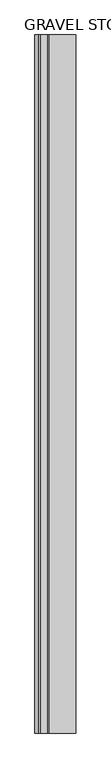
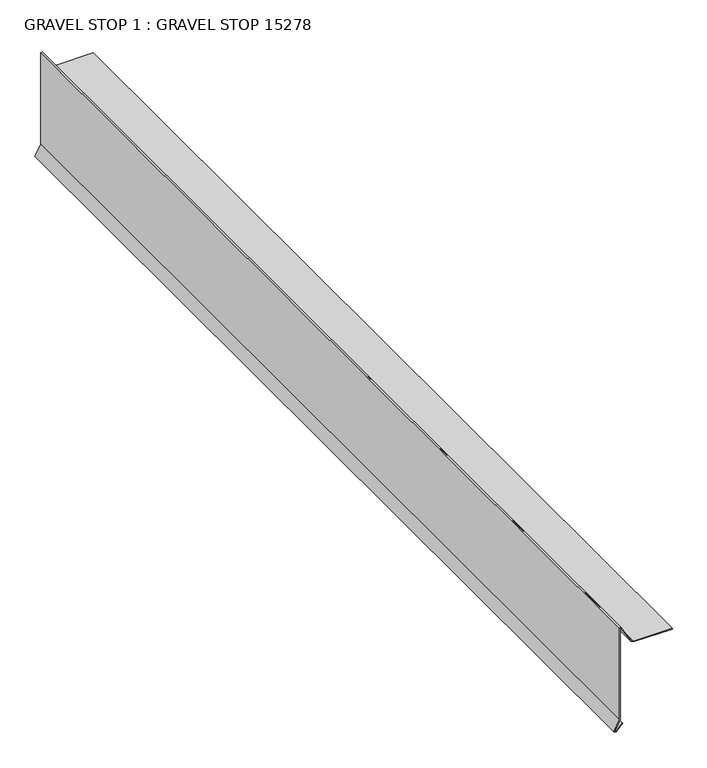
"""IFC4 building model written with IfcOpenShell, lengths in millimetres: proxy geometry, GRAVEL STOP 1 : GRAVEL STOP 15278."""

import ifcopenshell
import ifcopenshell.guid

model = None  # the IFC model being written
_history = None  # IfcOwnerHistory: only IFC2X3 demands one
_inside = {}  # id of a spatial element -> (the spatial element, [elements in it])
_under = {}  # id of a project, library or spatial element -> (it, [spatial elements below it])
_declared = {}  # id of a project -> (the project, [libraries it declares])
_typed = {}  # id of a type object -> (the type object, [elements of that type])
_made_of = {}  # id of a material, layer set ... -> (it, [elements and type objects made of it])


def new_model(schema):
    """Start an empty IFC model of exactly this schema.

    Asked for "IFC4X3", IfcOpenShell would pick the latest addendum, in which some entities
    have other attributes; the version numbers below select the first issue.
    IFC2X3 requires an IfcOwnerHistory on every rooted entity: one is made here for all.
    """
    global model, _history
    if schema == "IFC4X3":
        model = ifcopenshell.file(schema_version=(4, 3, 0, 0))
    else:
        model = ifcopenshell.file(schema=schema)
    _inside.clear()
    _under.clear()
    _declared.clear()
    _typed.clear()
    _made_of.clear()
    _history = None
    if model.schema == "IFC2X3":
        org = make("IfcOrganization", Name="unknown")
        user = make(
            "IfcPersonAndOrganization",
            ThePerson=make("IfcPerson", FamilyName="unknown"),
            TheOrganization=org,
        )
        app = make(
            "IfcApplication",
            ApplicationDeveloper=org,
            Version="unknown",
            ApplicationFullName="unknown",
            ApplicationIdentifier="unknown",
        )
        _history = make(
            "IfcOwnerHistory",
            OwningUser=user,
            OwningApplication=app,
            ChangeAction="ADDED",
            CreationDate=0,
        )
    return model


def make(cls, **values):
    """One entity of the class cls with the attributes given. An attribute that is None is left unset."""
    return model.create_entity(
        cls, **{name: value for name, value in values.items() if value is not None}
    )


def rooted(cls, **values):
    """An entity with a GlobalId (a new one), such as an element, a storey or a relation."""
    return make(cls, GlobalId=ifcopenshell.guid.new(), OwnerHistory=_history, **values)


def si_unit(unit_type, name, prefix=None):
    """IfcSIUnit, for example si_unit("LENGTHUNIT", "METRE", prefix="MILLI")."""
    return make("IfcSIUnit", UnitType=unit_type, Prefix=prefix, Name=name)


def assignment(units):
    """IfcUnitAssignment: the units of a project."""
    return None if units is None else make("IfcUnitAssignment", Units=units)


def point(xyz):
    """IfcCartesianPoint."""
    return None if xyz is None else make("IfcCartesianPoint", Coordinates=xyz)


def direction(xyz):
    """IfcDirection."""
    return None if xyz is None else make("IfcDirection", DirectionRatios=xyz)


def frame(location, z_axis=None, x_axis=None):
    """IfcAxis2Placement3D, a coordinate frame: its origin and axes. An axis left out is left unset."""
    return make(
        "IfcAxis2Placement3D",
        Location=point(location),
        Axis=direction(z_axis),
        RefDirection=direction(x_axis),
    )


def origin():
    """The frame at (0, 0, 0) with its axes left unset."""
    return frame((0.0, 0.0, 0.0))


def place(relative_to, where):
    """IfcLocalPlacement: puts the frame where relative to a parent placement (None: the world)."""
    return make(
        "IfcLocalPlacement", PlacementRelTo=relative_to, RelativePlacement=where
    )


def context(
    kind, dimensions, precision=None, world=None, true_north=None, identifier=None
):
    """IfcGeometricRepresentationContext, for example the 3D "Model" context."""
    return make(
        "IfcGeometricRepresentationContext",
        ContextIdentifier=identifier,
        ContextType=kind,
        CoordinateSpaceDimension=dimensions,
        Precision=precision,
        WorldCoordinateSystem=world,
        TrueNorth=true_north,
    )


def project(units=None, contexts=None):
    """IfcProject with its units and contexts."""
    return rooted(
        "IfcProject",
        Name="project",
        RepresentationContexts=contexts,
        UnitsInContext=assignment(units),
    )


def spatial(cls, under=None, at=None, **own):
    """A site, building, storey or space (cls), placed at a placement, below another one or the project."""
    s = rooted(cls, ObjectPlacement=at, **own)
    if under is not None:
        _under.setdefault(under.id(), (under, []))[1].append(s)
    return s


def polyline(points):
    """IfcPolyline through the points."""
    return make("IfcPolyline", Points=[point(p) for p in points])


def outline(outer, holes=None, kind="AREA"):
    """IfcArbitraryClosedProfileDef: a profile drawn as a closed curve; with holes, ...WithVoids."""
    if holes is None:
        return make("IfcArbitraryClosedProfileDef", ProfileType=kind, OuterCurve=outer)
    return make(
        "IfcArbitraryProfileDefWithVoids",
        ProfileType=kind,
        OuterCurve=outer,
        InnerCurves=holes,
    )


def extrude(swept, where, along, depth):
    """IfcExtrudedAreaSolid: the profile swept, set in the frame where, extruded along a direction by depth."""
    return make(
        "IfcExtrudedAreaSolid",
        SweptArea=swept,
        Position=where,
        ExtrudedDirection=direction(along),
        Depth=depth,
    )


def shape(context_of_items, identifier, shape_type, items):
    """IfcShapeRepresentation: the items that make up one representation, for example the "Body"."""
    return make(
        "IfcShapeRepresentation",
        ContextOfItems=context_of_items,
        RepresentationIdentifier=identifier,
        RepresentationType=shape_type,
        Items=items,
    )


def source(mapping_origin, context_of_items, identifier, shape_type, items):
    """IfcRepresentationMap: a shape defined once, which mapped items show again and again."""
    return make(
        "IfcRepresentationMap",
        MappingOrigin=mapping_origin,
        MappedRepresentation=shape(context_of_items, identifier, shape_type, items),
    )


def transform(
    local_origin,
    x_axis=None,
    y_axis=None,
    z_axis=None,
    scale=None,
    scale2=None,
    scale3=None,
    uniform=True,
):
    """IfcCartesianTransformationOperator3D, or its non-uniform kind. x_axis, y_axis, z_axis: its Axis1, 2, 3."""
    if uniform:
        return make(
            "IfcCartesianTransformationOperator3D",
            Axis1=direction(x_axis),
            Axis2=direction(y_axis),
            LocalOrigin=point(local_origin),
            Scale=scale,
            Axis3=direction(z_axis),
        )
    return make(
        "IfcCartesianTransformationOperator3DnonUniform",
        Axis1=direction(x_axis),
        Axis2=direction(y_axis),
        LocalOrigin=point(local_origin),
        Scale=scale,
        Axis3=direction(z_axis),
        Scale2=scale2,
        Scale3=scale3,
    )


def mapped(mapping_source, mapping_target):
    """IfcMappedItem: shows the shape of a source again, moved by a transform."""
    return make(
        "IfcMappedItem", MappingSource=mapping_source, MappingTarget=mapping_target
    )


def made_of(thing, what):
    """Note that an element or type object is made of a material, layer set ...; save() writes the relation."""
    if what is not None:
        _made_of.setdefault(what.id(), (what, []))[1].append(thing)
    return thing


def element(
    cls,
    number,
    at=None,
    inside=None,
    cuts=None,
    type_object=None,
    material=None,
    context=None,
    identifier="Body",
    shape_type=None,
    held_by="IfcProductDefinitionShape",
    body=None,
    shapes=None,
    **own,
):
    """One element of the class cls, such as IfcWall. Its Tag is "e" and its number.

    at: its placement. inside: the storey or other place that contains it. cuts: it is an
    opening in that element (IfcRelVoidsElement). A single representation is given by context,
    identifier, shape_type and body (its items); several are given by shapes. held_by: the class
    of the entity that holds the representations. save() writes the other relations.
    """
    e = rooted(cls, Tag="e%d" % number, ObjectPlacement=at, **own)
    if body is not None:
        shapes = [shape(context, identifier, shape_type, body)]
    if shapes is not None:
        e.Representation = make(held_by, Representations=shapes)
    if inside is not None:
        _inside.setdefault(inside.id(), (inside, []))[1].append(e)
    if cuts is not None:
        rooted(
            "IfcRelVoidsElement", RelatingBuildingElement=cuts, RelatedOpeningElement=e
        )
    if type_object is not None:
        _typed.setdefault(type_object.id(), (type_object, []))[1].append(e)
    return made_of(e, material)


def aggregate(whole, parts):
    """IfcRelAggregates: a whole, such as a stair, and the parts it consists of."""
    return rooted("IfcRelAggregates", RelatingObject=whole, RelatedObjects=parts)


def save(model, path):
    """Write the relations noted so far, then the file.

    IfcRelAggregates (storeys below a building ...), IfcRelContainedInSpatialStructure (elements
    in a storey), IfcRelDefinesByType, IfcRelAssociatesMaterial and IfcRelDeclares: one each for
    every whole, place, type object, material and project.
    """
    for whole, parts in _under.values():
        aggregate(whole, parts)
    for where, things in _inside.values():
        rooted(
            "IfcRelContainedInSpatialStructure",
            RelatedElements=things,
            RelatingStructure=where,
        )
    for kind, things in _typed.values():
        rooted("IfcRelDefinesByType", RelatedObjects=things, RelatingType=kind)
    for what, things in _made_of.values():
        rooted("IfcRelAssociatesMaterial", RelatedObjects=things, RelatingMaterial=what)
    for by, libraries in _declared.values():
        rooted("IfcRelDeclares", RelatingContext=by, RelatedDefinitions=libraries)
    model.write(path)


def gravel_stop_1_gravel_stop_15278_885a835c(model_context):
    return source(origin(), model_context, "Body", "SweptSolid", [
        extrude(outline(polyline([(40077.410403, -2814.9855343), (40091.8049, -2800.5910374), (40092.8027062, -2801.5888435), (40079.2807815, -2815.1107682), (40080.9054201, -2817.2404183), (40101.495749, -2805.9993985), (40293.447969, -2805.9993985), (40293.699878, -2805.0592614), (40258.5078708, -2784.7411466), (40255.9633674, -2780.3339375), (40255.9633674, -2702.4979247), (40257.3744784, -2702.4979247), (40257.3744784, -2779.9558314), (40259.5408757, -2783.7081416), (40295.3431515, -2804.3785952), (40294.5307525, -2807.4105095), (40101.8558531, -2807.4105095), (40080.5182783, -2819.0594785), (40077.410403, -2814.9855343)])), frame((0.0, -1052.8906573, 0.0), z_axis=(0.0, 1.0, 0.0), x_axis=(0.0, 0.0, 1.0)), (0.0, 0.0, 1.0), 2000.25),
    ])


if __name__ == "__main__":
    model = new_model("IFC4")
    model_context = context("Model", 3, world=origin())
    ifc_project = project(units=[si_unit("LENGTHUNIT", "METRE", prefix="MILLI")], contexts=[model_context])
    site = spatial("IfcSite", under=ifc_project)
    building = spatial("IfcBuilding", under=site)
    placement = place(None, origin())
    gravel_stop_1_gravel_stop_15278_shape = gravel_stop_1_gravel_stop_15278_885a835c(model_context)
    element("IfcBuildingElementProxy", 1, Name="GRAVEL STOP 1 : GRAVEL STOP 15278", ObjectType="GRAVEL STOP 1 : GRAVEL STOP 15278", at=placement, inside=building, context=model_context, shape_type="MappedRepresentation", body=[
        mapped(gravel_stop_1_gravel_stop_15278_shape, transform((0.0, 0.0, 0.0), x_axis=(1.0, 0.0, 0.0), y_axis=(0.0, 1.0, 0.0), z_axis=(0.0, 0.0, 1.0))),
    ])
    save(model, "model.ifc")

# Revit data of these elements
# Type "GRAVEL STOP 1 : GRAVEL STOP 15278"
#   NameOverride = "GRAVEL STOP"
# Element 1 (IfcBuildingElementProxy, "GRAVEL STOP 1 : GRAVEL STOP 15278")
#   Materials on its faces: "GRAVEL STOP REQUIRED WITH GRAVEL SURFACE SYSTEMS"
# Materials
#   "GRAVEL STOP REQUIRED WITH GRAVEL SURFACE SYSTEMS": class "Unassigned", colour RGB 170 170 127, transparency 0, Cost = 0
